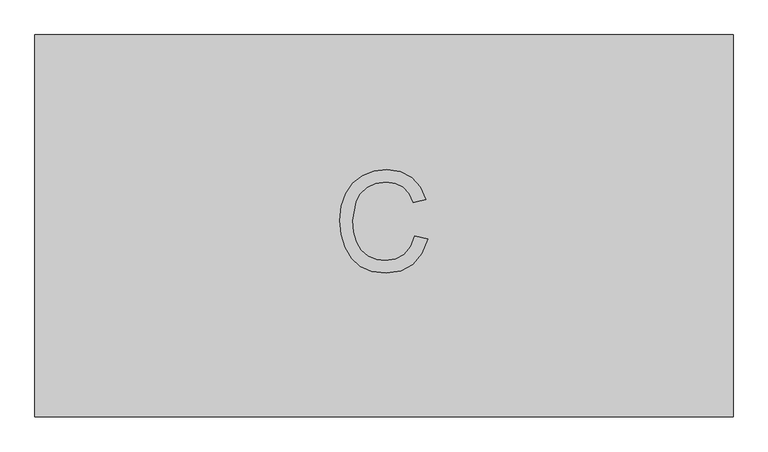
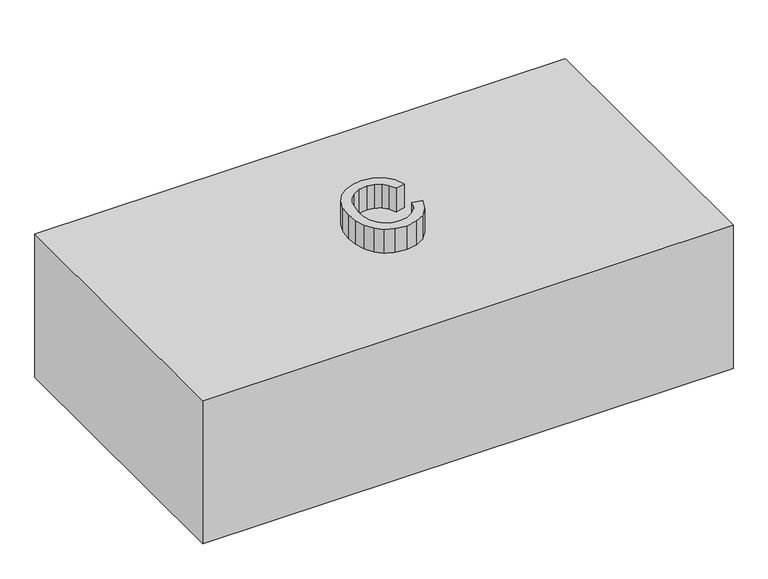
"""IFC4 building model written with IfcOpenShell, lengths in millimetres: proxy geometry, The Messy Family C : The Messy Family C."""

from ifc_helpers import new_model, si_unit, frame, origin, origin_with_axes, place, context, project, spatial, polyline, outline, extrude, source, transform, mapped, element, save


def generic_models_3b6b937a(model_context):
    return source(origin(), model_context, "Body", "SweptSolid", [
        extrude(outline(polyline([(541.9415527, 284.565081), (541.9415527, -299.634919), (-524.8584473, -299.634919), (-524.8584473, 284.565081), (541.9415527, 284.565081)])), origin_with_axes(), (0.0, 0.0, 1.0), 304.8),
        extrude(outline(polyline([(55.8849188, -22.8350413), (75.0218459, -27.7687803), (66.1915743, -50.06872), (52.3341218, -66.3603374), (34.1316149, -76.3259295), (12.2661807, -79.6477936), (-9.9309728, -77.134203), (-27.5588111, -69.5934315), (-41.0705282, -57.2871166), (-50.9193178, -40.4768959), (-56.9323122, -20.7139073), (-58.9366437, 0.4507118), (-56.6706746, 22.774012), (-49.8727671, 42.0511021), (-38.8980011, 57.6699369), (-24.1014561, 69.018471), (-6.5530435, 75.9285089), (12.6773256, 78.2318549), (33.6597327, 75.2510542), (51.007245, 66.3086523), (64.1778987, 51.955957), (72.62973, 32.7442762), (53.4928029, 28.1843053), (46.858419, 42.139872), (37.7945424, 51.7130077), (26.1890427, 57.2494478), (11.9297894, 59.0949278), (-4.5066631, 57.0485474), (-18.009036, 50.9094063), (-28.2549542, 41.3222543), (-34.9220428, 28.9318416), (-39.7997166, 0.4880886), (-38.3560373, -17.1911429), (-34.0249994, -32.4782584), (-26.6430793, -44.7892455), (-16.0467534, -53.5400913), (-3.3433099, -58.7681727), (10.3599633, -60.5108665), (26.3338778, -58.137439), (39.6446945, -51.0171566), (49.6943845, -39.2247728), (55.8849188, -22.8350413)])), frame((0.0, 0.0, 304.8), z_axis=(0.0, 0.0, 1.0), x_axis=(1.0, 0.0, 0.0)), (0.0, 0.0, 1.0), 50.8),
    ])


if __name__ == "__main__":
    model = new_model("IFC4")
    model_context = context("Model", 3, world=origin())
    ifc_project = project(units=[si_unit("LENGTHUNIT", "METRE", prefix="MILLI")], contexts=[model_context])
    site = spatial("IfcSite", under=ifc_project)
    building = spatial("IfcBuilding", under=site)
    placement = place(None, origin())
    generic_models_shape = generic_models_3b6b937a(model_context)
    element("IfcBuildingElementProxy", 1, Name="The Messy Family C : The Messy Family C", ObjectType="The Messy Family C : The Messy Family C", at=placement, inside=building, context=model_context, shape_type="MappedRepresentation", body=[
        mapped(generic_models_shape, transform((0.0, 0.0, 0.0), x_axis=(1.0, 0.0, 0.0), y_axis=(0.0, 1.0, 0.0), z_axis=(0.0, 0.0, 1.0))),
    ])
    save(model, "model.ifc")

# Revit data of these elements
# Type "The Messy Family C : The Messy Family C"
#   TBC-Parameter 2 = ""
#   TBC-Parameter 1 = ""
#   Other Company Parameter 2 = ""
#   Other Company Parameter 1 = ""
#   TBC-Parameter 3 = 2' - 0"
#   Other Company Parameter 3 = 1' - 0"
#   Default Elevation = 0
